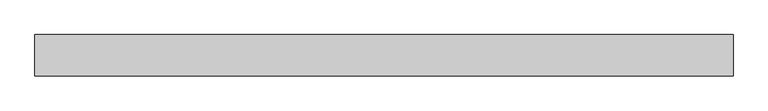
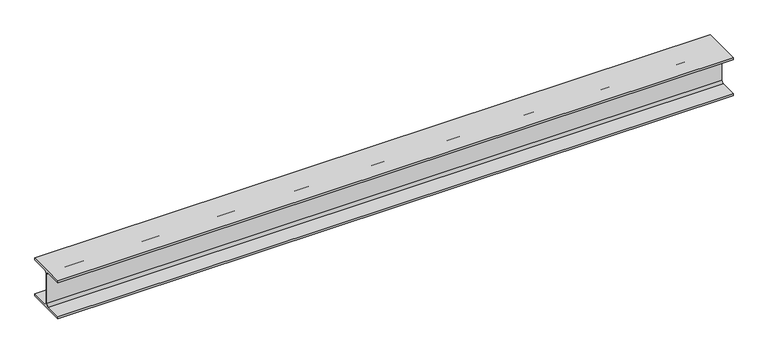
"""IFC4 building model written with IfcOpenShell, lengths in millimetres: beam geometry, 0912_Steel Framing_H-KSD3502 : H_SB_ASB_H-300x300x10x15."""

from ifc_helpers import new_model, si_unit, point, frame, frame_2d, origin, place, context, project, spatial, polyline, circle_curve, trimmed, segment, composite_curve, outline, extrude, source, transform, mapped, element, save


def beam_61bab96b(model_context):
    return source(origin(), model_context, "Body", "SweptSolid", [
        extrude(outline(composite_curve([segment(polyline([(150.0, -135.0), (150.0, -150.0), (-150.0, -150.0), (-150.0, -135.0), (-23.0, -135.0)]), True, "CONTINUOUS"), segment(trimmed(circle_curve(frame_2d((-23.0, -117.0)), 18.0), [point((-23.0, -135.0))], [point((-5.0, -117.0))], True, "CARTESIAN"), True, "CONTINUOUS"), segment(polyline([(-5.0, -117.0), (-5.0, 117.0)]), True, "CONTINUOUS"), segment(trimmed(circle_curve(frame_2d((-23.0, 117.0)), 18.0), [point((-5.0, 117.0))], [point((-23.0, 135.0))], True, "CARTESIAN"), True, "CONTINUOUS"), segment(polyline([(-23.0, 135.0), (-150.0, 135.0), (-150.0, 150.0), (150.0, 150.0), (150.0, 135.0), (23.0, 135.0)]), True, "CONTINUOUS"), segment(trimmed(circle_curve(frame_2d((23.0, 117.0)), 18.0), [point((23.0, 135.0))], [point((5.0, 117.0))], True, "CARTESIAN"), True, "CONTINUOUS"), segment(polyline([(5.0, 117.0), (5.0, -117.0)]), True, "CONTINUOUS"), segment(trimmed(circle_curve(frame_2d((23.0, -117.0)), 18.0), [point((5.0, -117.0))], [point((23.0, -135.0))], True, "CARTESIAN"), True, "CONTINUOUS"), segment(polyline([(23.0, -135.0), (150.0, -135.0)]), True, "CONTINUOUS")], self_intersect=False)), frame((-2413.6981883, 0.0, 0.0), z_axis=(1.0, 0.0, 0.0), x_axis=(0.0, 1.0, 0.0)), (0.0, 0.0, 1.0), 5076.9152279),
    ])


if __name__ == "__main__":
    model = new_model("IFC4")
    model_context = context("Model", 3, world=origin())
    ifc_project = project(units=[si_unit("LENGTHUNIT", "METRE", prefix="MILLI")], contexts=[model_context])
    site = spatial("IfcSite", under=ifc_project)
    building = spatial("IfcBuilding", under=site)
    placement = place(None, origin())
    beam_shape = beam_61bab96b(model_context)
    element("IfcBeam", 1, ObjectType="0912_Steel Framing_H-KSD3502 : H_SB_ASB_H-300x300x10x15", at=placement, inside=building, context=model_context, shape_type="MappedRepresentation", body=[
        mapped(beam_shape, transform((0.0, 0.0, 0.0), x_axis=(1.0, 0.0, 0.0), y_axis=(0.0, 1.0, 0.0), z_axis=(0.0, 0.0, 1.0))),
    ])
    save(model, "model.ifc")

# Revit data of these elements
# Type "0912_Steel Framing_H-KSD3502 : H_SB_ASB_H-300x300x10x15"
#   H_WM Code_1 = "S01AA001-00001 | Main Steel Structure Fabrication Work | Shelter/Building | Heavy Steel - Standard (Weight≥90KG/M) | Material: (   )"
#   H_WM Code_2 = "S03AA027-00001 | Main Steel Structure Erection Work | Shelter/Building | Heavy Steel (Weight≥90KG/M) | Material: (   )"
#   H_WM Code_3 = "S01AA010-00001 | Main Steel Structure Fabrication Work | Shelter/Building | Steel Painting/Coating | for Non-Fireproofed Steel Surface, Surface Preparation, Primer, Second & Final Coat | Material: (   )"
#   H_Q'ty Cal Type Tag = "SB-Q2"
#   Width = 30.0 cm
#   Web Thickness = 1.0 cm
#   Web Fillet = 1.8 cm
#   Warping Constant = 1370000.0 cm⁶
#   W = 0
#   Torsional Moment of Inertia = 77.00 cm⁴
#   Section Area = 119.8 cm²
#   Plastic Modulus weak axis = 684.0 cm³
#   Plastic Modulus strong axis = 1500.0 cm³
#   Perimeter = 1.75 m²/m
#   Nominal Weight = 94.00 kgf/m
#   Moment of Inertia weak axis = 6750.00 cm⁴
#   Moment of Inertia strong axis = 20400.00 cm⁴
#   Height = 30.0 cm
#   Flange Thickness = 1.5 cm
#   Elastic Modulus weak axis = 450.0 cm³
#   Elastic Modulus strong axis = 1360.0 cm³
#   Centroid Vertical = 15.0 cm
#   Centroid Horizontal = 15.0 cm
#   Ix = 204000000
#   Length [instance default] = 1.5240 m
#   Zx = 1500000
#   b = 0.3000 m
#   h = 0.3000 m
#   r = 0.0180 m
#   s = 0.0100 m
#   t = 0.0150 m
#   A = 0.01198 m²
#   Structural Material [instance default] = Steel, 45-345
#   Assembly Code = ""
# Element 1 (IfcBeam, "0912_Steel Framing_H-KSD3502 : H_SB_ASB_H-300x300x10x15")
#   Structural Material = none
# Materials
#   "Steel, 45-345": class "Metal", colour RGB 189 187 185, transparency 0, Description = "Steel 345 MPa", Cost = 0
